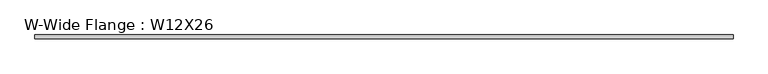
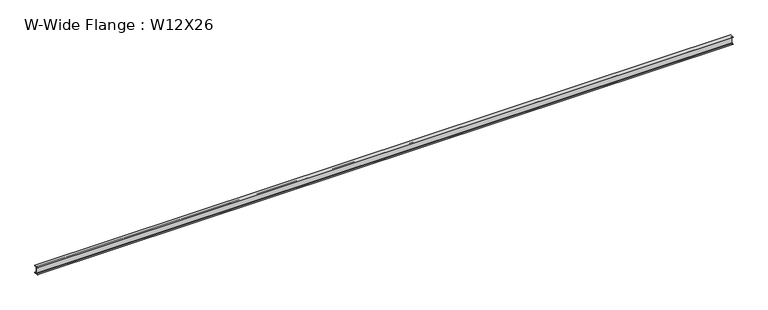
"""IFC4 building model written with IfcOpenShell, lengths in millimetres: beam geometry, W-Wide Flange : W12X26."""

from ifc_helpers import new_model, si_unit, point, frame, frame_2d, origin, place, context, project, spatial, polyline, circle_curve, trimmed, segment, composite_curve, outline, extrude, source, transform, mapped, element, save


def w_wide_flange_w12x26_164c45fe(model_context):
    return source(origin(), model_context, "Body", "SweptSolid", [
        extrude(outline(composite_curve([segment(polyline([(82.4011719, -145.5539063), (82.4011719, -155.178125), (-82.4011719, -155.178125), (-82.4011719, -145.5539063), (-20.2902344, -145.5539063)]), True, "CONTINUOUS"), segment(trimmed(circle_curve(frame_2d((-20.2902344, -128.190625)), 17.3632812), [point((-20.2902344, -145.5539063))], [point((-2.9269531, -128.190625))], True, "CARTESIAN"), True, "CONTINUOUS"), segment(polyline([(-2.9269531, -128.190625), (-2.9269531, 128.190625)]), True, "CONTINUOUS"), segment(trimmed(circle_curve(frame_2d((-20.2902344, 128.190625)), 17.3632812), [point((-2.9269531, 128.190625))], [point((-20.2902344, 145.5539062))], True, "CARTESIAN"), True, "CONTINUOUS"), segment(polyline([(-20.2902344, 145.5539062), (-82.4011719, 145.5539062), (-82.4011719, 155.178125), (82.4011719, 155.178125), (82.4011719, 145.5539062), (20.2902344, 145.5539062)]), True, "CONTINUOUS"), segment(trimmed(circle_curve(frame_2d((20.2902344, 128.190625)), 17.3632812), [point((20.2902344, 145.5539062))], [point((2.9269531, 128.190625))], True, "CARTESIAN"), True, "CONTINUOUS"), segment(polyline([(2.9269531, 128.190625), (2.9269531, -128.190625)]), True, "CONTINUOUS"), segment(trimmed(circle_curve(frame_2d((20.2902344, -128.190625)), 17.3632812), [point((2.9269531, -128.190625))], [point((20.2902344, -145.5539063))], True, "CARTESIAN"), True, "CONTINUOUS"), segment(polyline([(20.2902344, -145.5539063), (82.4011719, -145.5539063)]), True, "CONTINUOUS")], self_intersect=False)), frame((-14097.0, 0.0, 0.0), z_axis=(1.0, 0.0, 0.0), x_axis=(0.0, 1.0, 0.0)), (0.0, 0.0, 1.0), 28194.0),
    ])


if __name__ == "__main__":
    model = new_model("IFC4")
    model_context = context("Model", 3, world=origin())
    ifc_project = project(units=[si_unit("LENGTHUNIT", "METRE", prefix="MILLI")], contexts=[model_context])
    site = spatial("IfcSite", under=ifc_project)
    building = spatial("IfcBuilding", under=site)
    placement = place(None, origin())
    w_wide_flange_w12x26_shape = w_wide_flange_w12x26_164c45fe(model_context)
    element("IfcBeam", 1, ObjectType="W-Wide Flange : W12X26", at=placement, inside=building, context=model_context, shape_type="MappedRepresentation", body=[
        mapped(w_wide_flange_w12x26_shape, transform((0.0, 0.0, 0.0), x_axis=(1.0, 0.0, 0.0), y_axis=(0.0, 1.0, 0.0), z_axis=(0.0, 0.0, 1.0))),
    ])
    save(model, "model.ifc")

# Revit data of these elements
# Type "W-Wide Flange : W12X26"
#   Assembly Code = "B10"
#   W = 26
#   Length [instance default] = 5' - 0"
#   bf = 0' - 6 125/256"
#   d = 1' - 0 7/32"
#   k = 0' - 1 1/16"
#   k2 = 0' - 0 175/256"
#   tf = 0' - 0 97/256"
#   tw = 0' - 0 59/256"
#   A = 0.053125 SF
#   Structural Material [instance default] = none
